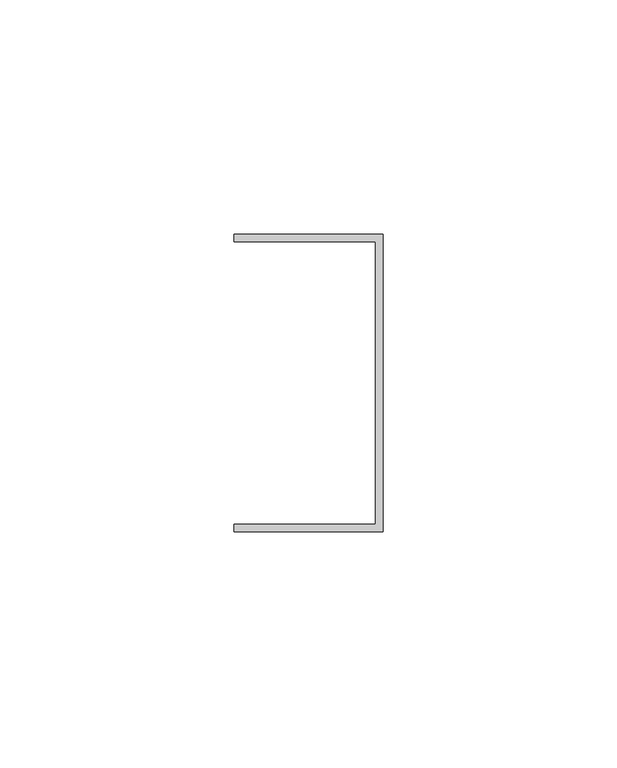
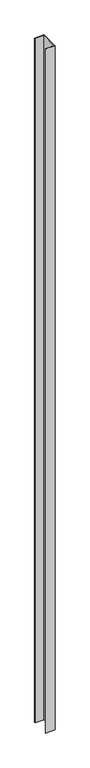
"""IFC4 building model written with IfcOpenShell, lengths in millimetres: proxy geometry, Generic Models 7:Generic Models 1:3:Generic Models 1:3 : Generic Models 7:Generic Models 1:305549:3:Generic Models 1:3:Generic Models 1:3 : Generic Models 7:Generic Models 1:305549:3 : Generic Models 7:Generic Models 1:3:Generic Models 1:3 : Generic Models 7:Generic Models 1:305549:301244:14 : Generic Models 7:Generic Models 1:3:Generic Models 1:3 : Generic Models 7:Generic Models 1:305549:3:Generic Models 1:3:Generic Models 1:3 : Generic Models 7:Generic Models 1:305549:3 : Generic Models 7:Generic Models 1:3:Generic Models 1:3 : Generic Models 7:Generic Models 1:305549:301244:308848."""

from ifc_helpers import new_model, si_unit, frame, origin, place, context, project, spatial, polyline, outline, extrude, source, transform, mapped, element, save


def generic_models_702f4d6f(model_context):
    return source(origin(), model_context, "Body", "SweptSolid", [
        extrude(outline(polyline([(570440.0912361, -579013.3913841), (570440.0912361, -579076.8913841), (570408.3412361, -579076.8913841), (570408.3412361, -579075.3038841), (570438.5037361, -579075.3038841), (570438.5037361, -579014.9788841), (570408.3412361, -579014.9788841), (570408.3412361, -579013.3913841), (570440.0912361, -579013.3913841)])), frame((0.0, 0.0, 3733.8), z_axis=(0.0, 0.0, 1.0), x_axis=(1.0, 0.0, 0.0)), (0.0, 0.0, 1.0), 2438.4),
    ])


if __name__ == "__main__":
    model = new_model("IFC4")
    model_context = context("Model", 3, world=origin())
    ifc_project = project(units=[si_unit("LENGTHUNIT", "METRE", prefix="MILLI")], contexts=[model_context])
    site = spatial("IfcSite", under=ifc_project)
    building = spatial("IfcBuilding", under=site)
    placement = place(None, origin())
    generic_models_shape = generic_models_702f4d6f(model_context)
    element("IfcBuildingElementProxy", 1, Name="Generic Models 7:Generic Models 1:3:Generic Models 1:3 : Generic Models 7:Generic Models 1:305549:3:Generic Models 1:3:Generic Models 1:3 : Generic Models 7:Generic Models 1:305549:3 : Generic Models 7:Generic Models 1:3:Generic Models 1:3 : Generic Models 7:Generic Models 1:305549:301244:14 : Generic Models 7:Generic Models 1:3:Generic Models 1:3 : Generic Models 7:Generic Models 1:305549:3:Generic Models 1:3:Generic Models 1:3 : Generic Models 7:Generic Models 1:305549:3 : Generic Models 7:Generic Models 1:3:Generic Models 1:3 : Generic Models 7:Generic Models 1:305549:301244:308848", ObjectType="Generic Models 7:Generic Models 1:3:Generic Models 1:3 : Generic Models 7:Generic Models 1:305549:3:Generic Models 1:3:Generic Models 1:3 : Generic Models 7:Generic Models 1:305549:3 : Generic Models 7:Generic Models 1:3:Generic Models 1:3 : Generic Models 7:Generic Models 1:305549:301244:14 : Generic Models 7:Generic Models 1:3:Generic Models 1:3 : Generic Models 7:Generic Models 1:305549:3:Generic Models 1:3:Generic Models 1:3 : Generic Models 7:Generic Models 1:305549:3 : Generic Models 7:Generic Models 1:3:Generic Models 1:3 : Generic Models 7:Generic Models 1:305549:301244:308848", at=placement, inside=building, context=model_context, shape_type="MappedRepresentation", body=[
        mapped(generic_models_shape, transform((0.0, 0.0, 0.0), x_axis=(1.0, 0.0, 0.0), y_axis=(0.0, 1.0, 0.0), z_axis=(0.0, 0.0, 1.0))),
    ])
    save(model, "model.ifc")

# Revit data of these elements
# Type "Generic Models 7:Generic Models 1:3:Generic Models 1:3 : Generic Models 7:Generic Models 1:305549:3:Generic Models 1:3:Generic Models 1:3 : Generic Models 7:Generic Models 1:305549:3 : Generic Models 7:Generic Models 1:3:Generic Models 1:3 : Generic Models 7:Generic Models 1:305549:301244:14 : Generic Models 7:Generic Models 1:3:Generic Models 1:3 : Generic Models 7:Generic Models 1:305549:3:Generic Models 1:3:Generic Models 1:3 : Generic Models 7:Generic Models 1:305549:3 : Generic Models 7:Generic Models 1:3:Generic Models 1:3 : Generic Models 7:Generic Models 1:305549:301244:308848"
#   NameOverride = "Generic Models 7:Generic Models 1:3:Generic Models 1:3 : Generic Models 7:Generic Models 1:305549:3:Generic Models 1:3:Generic Models 1:3 : Generic Models 7:Generic Models 1:305549:3 : Generic Models 7:Generic Models 1:3:Generic Models 1:3 : Generic Models 7:Generic Models 1:305549:301244:308848"
#   ObjectTypeOverride = "Generic Models 1:3:Generic Models 1:3 : Generic Models 7:Generic Models 1:305549:3 : Generic Models 7:Generic Models 1:3:Generic Models 1:3 : Generic Models 7:Generic Models 1:305549:301244"
#   Reference = "Generic Models 1"
#   Tag = "308848"
# Element 1 (IfcBuildingElementProxy, "Generic Models 7:Generic Models 1:3:Generic Models 1:3 : Generic Models 7:Generic Models 1:305549:3:Generic Models 1:3:Generic Models 1:3 : Generic Models 7:Generic Models 1:305549:3 : Generic Models 7:Generic Models 1:3:Generic Models 1:3 : Generic Models 7:Generic Models 1:305549:301244:14 : Generic Models 7:Generic Models 1:3:Generic Models 1:3 : Generic Models 7:Generic Models 1:305549:3:Generic Models 1:3:Generic Models 1:3 : Generic Models 7:Generic Models 1:305549:3 : Generic Models 7:Generic Models 1:3:Generic Models 1:3 : Generic Models 7:Generic Models 1:305549:301244:308848")
#   Materials on its faces: "GALVANIZED U-CHANNEL (250T125-33)"
# Materials
#   "GALVANIZED U-CHANNEL (250T125-33)": class "Unassigned", colour RGB 202 201 200, transparency 0, Keynote = "M05451300.02", Cost = 0
